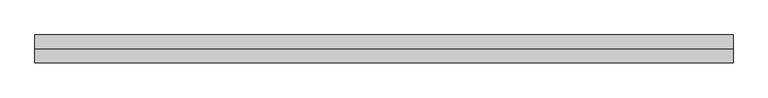
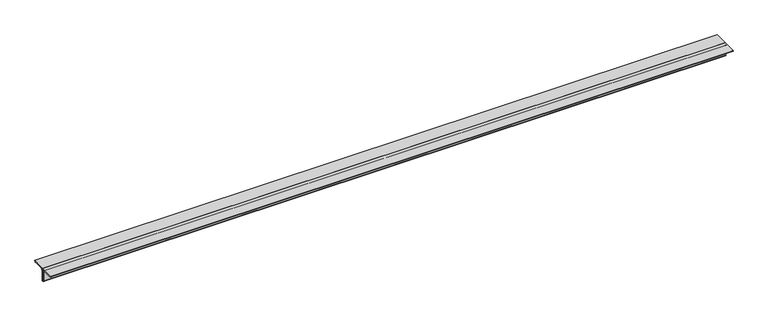
"""IFC4 building model written with IfcOpenShell, lengths in millimetres: member geometry, Steel Framing_2Ls_KS : H_SB_AR_S02_2Ls-100x100x10_VBR1."""

from ifc_helpers import new_model, si_unit, point, frame, frame_2d, origin, place, context, project, spatial, polyline, circle_curve, trimmed, segment, composite_curve, outline, extrude, source, transform, mapped, element, save


def member_efb42dbc(model_context):
    return source(origin(), model_context, "Body", "SweptSolid", [
        extrude(outline(composite_curve([segment(polyline([(0.0, 28.2), (100.0, 28.2)]), True, "CONTINUOUS"), segment(trimmed(circle_curve(frame_2d((90.0, 28.2)), 10.0), [point((100.0, 28.2))], [point((90.0, 18.2))], False, "CARTESIAN"), True, "CONTINUOUS"), segment(polyline([(90.0, 18.2), (20.0, 18.2)]), True, "CONTINUOUS"), segment(trimmed(circle_curve(frame_2d((20.0, 8.2)), 10.0), [point((20.0, 18.2))], [point((10.0, 8.2))], True, "CARTESIAN"), True, "CONTINUOUS"), segment(polyline([(10.0, 8.2), (10.0, -61.8)]), True, "CONTINUOUS"), segment(trimmed(circle_curve(frame_2d((0.0, -61.8)), 10.0), [point((10.0, -61.8))], [point((0.0, -71.8))], False, "CARTESIAN"), True, "CONTINUOUS"), segment(polyline([(0.0, -71.8), (0.0, 28.2)]), True, "CONTINUOUS")], self_intersect=False)), frame((-2600.492603, 0.0, 0.0), z_axis=(1.0, 0.0, 0.0), x_axis=(0.0, 1.0, 0.0)), (0.0, 0.0, 1.0), 4992.4085104),
        extrude(outline(composite_curve([segment(polyline([(0.0, 28.2), (0.0, -71.8)]), True, "CONTINUOUS"), segment(trimmed(circle_curve(frame_2d((0.0, -61.8)), 10.0), [point((0.0, -71.8))], [point((-10.0, -61.8))], False, "CARTESIAN"), True, "CONTINUOUS"), segment(polyline([(-10.0, -61.8), (-10.0, 8.2)]), True, "CONTINUOUS"), segment(trimmed(circle_curve(frame_2d((-20.0, 8.2)), 10.0), [point((-10.0, 8.2))], [point((-20.0, 18.2))], True, "CARTESIAN"), True, "CONTINUOUS"), segment(polyline([(-20.0, 18.2), (-90.0, 18.2)]), True, "CONTINUOUS"), segment(trimmed(circle_curve(frame_2d((-90.0, 28.2)), 10.0), [point((-90.0, 18.2))], [point((-100.0, 28.2))], False, "CARTESIAN"), True, "CONTINUOUS"), segment(polyline([(-100.0, 28.2), (0.0, 28.2)]), True, "CONTINUOUS")], self_intersect=False)), frame((-2600.492603, 0.0, 0.0), z_axis=(1.0, 0.0, 0.0), x_axis=(0.0, 1.0, 0.0)), (0.0, 0.0, 1.0), 4992.4085104),
    ])


if __name__ == "__main__":
    model = new_model("IFC4")
    model_context = context("Model", 3, world=origin())
    ifc_project = project(units=[si_unit("LENGTHUNIT", "METRE", prefix="MILLI")], contexts=[model_context])
    site = spatial("IfcSite", under=ifc_project)
    building = spatial("IfcBuilding", under=site)
    placement = place(None, origin())
    member_shape = member_efb42dbc(model_context)
    element("IfcMember", 1, ObjectType="Steel Framing_2Ls_KS : H_SB_AR_S02_2Ls-100x100x10_VBR1", at=placement, inside=building, context=model_context, shape_type="MappedRepresentation", body=[
        mapped(member_shape, transform((0.0, 0.0, 0.0), x_axis=(1.0, 0.0, 0.0), y_axis=(0.0, 1.0, 0.0), z_axis=(0.0, 0.0, 1.0))),
    ])
    save(model, "model.ifc")

# Revit data of these elements
# Type "Steel Framing_2Ls_KS : H_SB_AR_S02_2Ls-100x100x10_VBR1"
#   Type Comments = "MAIN"
#   Type Mark = "VBR1"
#   H_SectionID = "2Ls-100x100x10"
#   Assembly Code = "B10"
#   Legs = "LLBB"
#   H_Ratio for Additional Steel Plate = 0.2
#   W = 0
#   Perimeter = 0.80 m²/m
#   Nominal Weight = 29.80 kgf/m
#   Length [instance default] = 1524 mm
#   Space = 0 mm
#   b = 100 mm
#   d = 100 mm
#   t = 10 mm
#   y = 28.2 mm
#   A = 0.0038 m²
#   Structural Material [instance default] = Steel, 45-345
# Element 1 (IfcMember, "Steel Framing_2Ls_KS : H_SB_AR_S02_2Ls-100x100x10_VBR1")
#   Materials on its faces: "Steel, 45-345"
# Materials
#   "Steel, 45-345": class "Metal", colour RGB 189 187 185, transparency 0, Description = "Steel 345 MPa", Cost = 0
